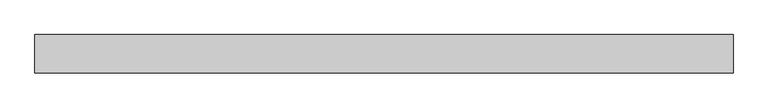
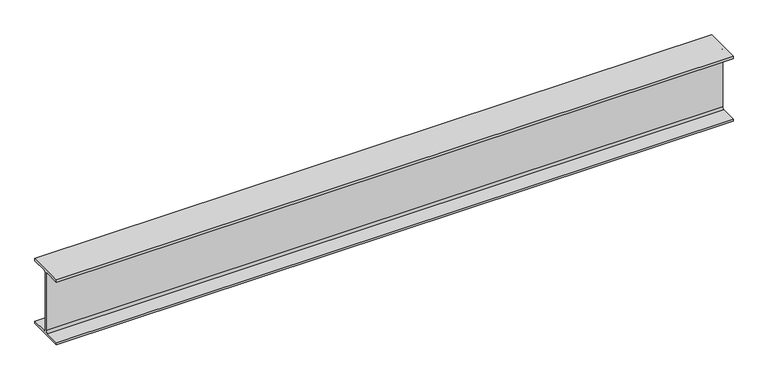
"""IFC4 building model written with IfcOpenShell, lengths in millimetres: beam geometry, Steel Beam_H-KSD3502 : H_SB_ASB_H-250x125x6x9."""

import ifcopenshell
import ifcopenshell.guid

model = None  # the IFC model being written
_history = None  # IfcOwnerHistory: only IFC2X3 demands one
_inside = {}  # id of a spatial element -> (the spatial element, [elements in it])
_under = {}  # id of a project, library or spatial element -> (it, [spatial elements below it])
_declared = {}  # id of a project -> (the project, [libraries it declares])
_typed = {}  # id of a type object -> (the type object, [elements of that type])
_made_of = {}  # id of a material, layer set ... -> (it, [elements and type objects made of it])


def new_model(schema):
    """Start an empty IFC model of exactly this schema.

    Asked for "IFC4X3", IfcOpenShell would pick the latest addendum, in which some entities
    have other attributes; the version numbers below select the first issue.
    IFC2X3 requires an IfcOwnerHistory on every rooted entity: one is made here for all.
    """
    global model, _history
    if schema == "IFC4X3":
        model = ifcopenshell.file(schema_version=(4, 3, 0, 0))
    else:
        model = ifcopenshell.file(schema=schema)
    _inside.clear()
    _under.clear()
    _declared.clear()
    _typed.clear()
    _made_of.clear()
    _history = None
    if model.schema == "IFC2X3":
        org = make("IfcOrganization", Name="unknown")
        user = make(
            "IfcPersonAndOrganization",
            ThePerson=make("IfcPerson", FamilyName="unknown"),
            TheOrganization=org,
        )
        app = make(
            "IfcApplication",
            ApplicationDeveloper=org,
            Version="unknown",
            ApplicationFullName="unknown",
            ApplicationIdentifier="unknown",
        )
        _history = make(
            "IfcOwnerHistory",
            OwningUser=user,
            OwningApplication=app,
            ChangeAction="ADDED",
            CreationDate=0,
        )
    return model


def make(cls, **values):
    """One entity of the class cls with the attributes given. An attribute that is None is left unset."""
    return model.create_entity(
        cls, **{name: value for name, value in values.items() if value is not None}
    )


def rooted(cls, **values):
    """An entity with a GlobalId (a new one), such as an element, a storey or a relation."""
    return make(cls, GlobalId=ifcopenshell.guid.new(), OwnerHistory=_history, **values)


def si_unit(unit_type, name, prefix=None):
    """IfcSIUnit, for example si_unit("LENGTHUNIT", "METRE", prefix="MILLI")."""
    return make("IfcSIUnit", UnitType=unit_type, Prefix=prefix, Name=name)


def assignment(units):
    """IfcUnitAssignment: the units of a project."""
    return None if units is None else make("IfcUnitAssignment", Units=units)


def point(xyz):
    """IfcCartesianPoint."""
    return None if xyz is None else make("IfcCartesianPoint", Coordinates=xyz)


def direction(xyz):
    """IfcDirection."""
    return None if xyz is None else make("IfcDirection", DirectionRatios=xyz)


def frame(location, z_axis=None, x_axis=None):
    """IfcAxis2Placement3D, a coordinate frame: its origin and axes. An axis left out is left unset."""
    return make(
        "IfcAxis2Placement3D",
        Location=point(location),
        Axis=direction(z_axis),
        RefDirection=direction(x_axis),
    )


def frame_2d(location, x_axis=None):
    """IfcAxis2Placement2D, a coordinate frame in the plane: its origin and x axis."""
    return make(
        "IfcAxis2Placement2D", Location=point(location), RefDirection=direction(x_axis)
    )


def origin():
    """The frame at (0, 0, 0) with its axes left unset."""
    return frame((0.0, 0.0, 0.0))


def place(relative_to, where):
    """IfcLocalPlacement: puts the frame where relative to a parent placement (None: the world)."""
    return make(
        "IfcLocalPlacement", PlacementRelTo=relative_to, RelativePlacement=where
    )


def context(
    kind, dimensions, precision=None, world=None, true_north=None, identifier=None
):
    """IfcGeometricRepresentationContext, for example the 3D "Model" context."""
    return make(
        "IfcGeometricRepresentationContext",
        ContextIdentifier=identifier,
        ContextType=kind,
        CoordinateSpaceDimension=dimensions,
        Precision=precision,
        WorldCoordinateSystem=world,
        TrueNorth=true_north,
    )


def project(units=None, contexts=None):
    """IfcProject with its units and contexts."""
    return rooted(
        "IfcProject",
        Name="project",
        RepresentationContexts=contexts,
        UnitsInContext=assignment(units),
    )


def spatial(cls, under=None, at=None, **own):
    """A site, building, storey or space (cls), placed at a placement, below another one or the project."""
    s = rooted(cls, ObjectPlacement=at, **own)
    if under is not None:
        _under.setdefault(under.id(), (under, []))[1].append(s)
    return s


def polyline(points):
    """IfcPolyline through the points."""
    return make("IfcPolyline", Points=[point(p) for p in points])


def circle_curve(where, radius):
    """IfcCircle in the frame where."""
    return make("IfcCircle", Position=where, Radius=radius)


def trimmed(basis, trim1, trim2, sense, master):
    """IfcTrimmedCurve: the piece of a basis curve between two trims."""
    return make(
        "IfcTrimmedCurve",
        BasisCurve=basis,
        Trim1=trim1,
        Trim2=trim2,
        SenseAgreement=sense,
        MasterRepresentation=master,
    )


def segment(curve, same_sense, transition):
    """IfcCompositeCurveSegment."""
    return make(
        "IfcCompositeCurveSegment",
        Transition=transition,
        SameSense=same_sense,
        ParentCurve=curve,
    )


def composite_curve(segments, self_intersect=None):
    """IfcCompositeCurve: segments joined end to end."""
    return make("IfcCompositeCurve", Segments=segments, SelfIntersect=self_intersect)


def outline(outer, holes=None, kind="AREA"):
    """IfcArbitraryClosedProfileDef: a profile drawn as a closed curve; with holes, ...WithVoids."""
    if holes is None:
        return make("IfcArbitraryClosedProfileDef", ProfileType=kind, OuterCurve=outer)
    return make(
        "IfcArbitraryProfileDefWithVoids",
        ProfileType=kind,
        OuterCurve=outer,
        InnerCurves=holes,
    )


def extrude(swept, where, along, depth):
    """IfcExtrudedAreaSolid: the profile swept, set in the frame where, extruded along a direction by depth."""
    return make(
        "IfcExtrudedAreaSolid",
        SweptArea=swept,
        Position=where,
        ExtrudedDirection=direction(along),
        Depth=depth,
    )


def shape(context_of_items, identifier, shape_type, items):
    """IfcShapeRepresentation: the items that make up one representation, for example the "Body"."""
    return make(
        "IfcShapeRepresentation",
        ContextOfItems=context_of_items,
        RepresentationIdentifier=identifier,
        RepresentationType=shape_type,
        Items=items,
    )


def source(mapping_origin, context_of_items, identifier, shape_type, items):
    """IfcRepresentationMap: a shape defined once, which mapped items show again and again."""
    return make(
        "IfcRepresentationMap",
        MappingOrigin=mapping_origin,
        MappedRepresentation=shape(context_of_items, identifier, shape_type, items),
    )


def transform(
    local_origin,
    x_axis=None,
    y_axis=None,
    z_axis=None,
    scale=None,
    scale2=None,
    scale3=None,
    uniform=True,
):
    """IfcCartesianTransformationOperator3D, or its non-uniform kind. x_axis, y_axis, z_axis: its Axis1, 2, 3."""
    if uniform:
        return make(
            "IfcCartesianTransformationOperator3D",
            Axis1=direction(x_axis),
            Axis2=direction(y_axis),
            LocalOrigin=point(local_origin),
            Scale=scale,
            Axis3=direction(z_axis),
        )
    return make(
        "IfcCartesianTransformationOperator3DnonUniform",
        Axis1=direction(x_axis),
        Axis2=direction(y_axis),
        LocalOrigin=point(local_origin),
        Scale=scale,
        Axis3=direction(z_axis),
        Scale2=scale2,
        Scale3=scale3,
    )


def mapped(mapping_source, mapping_target):
    """IfcMappedItem: shows the shape of a source again, moved by a transform."""
    return make(
        "IfcMappedItem", MappingSource=mapping_source, MappingTarget=mapping_target
    )


def made_of(thing, what):
    """Note that an element or type object is made of a material, layer set ...; save() writes the relation."""
    if what is not None:
        _made_of.setdefault(what.id(), (what, []))[1].append(thing)
    return thing


def element(
    cls,
    number,
    at=None,
    inside=None,
    cuts=None,
    type_object=None,
    material=None,
    context=None,
    identifier="Body",
    shape_type=None,
    held_by="IfcProductDefinitionShape",
    body=None,
    shapes=None,
    **own,
):
    """One element of the class cls, such as IfcWall. Its Tag is "e" and its number.

    at: its placement. inside: the storey or other place that contains it. cuts: it is an
    opening in that element (IfcRelVoidsElement). A single representation is given by context,
    identifier, shape_type and body (its items); several are given by shapes. held_by: the class
    of the entity that holds the representations. save() writes the other relations.
    """
    e = rooted(cls, Tag="e%d" % number, ObjectPlacement=at, **own)
    if body is not None:
        shapes = [shape(context, identifier, shape_type, body)]
    if shapes is not None:
        e.Representation = make(held_by, Representations=shapes)
    if inside is not None:
        _inside.setdefault(inside.id(), (inside, []))[1].append(e)
    if cuts is not None:
        rooted(
            "IfcRelVoidsElement", RelatingBuildingElement=cuts, RelatedOpeningElement=e
        )
    if type_object is not None:
        _typed.setdefault(type_object.id(), (type_object, []))[1].append(e)
    return made_of(e, material)


def aggregate(whole, parts):
    """IfcRelAggregates: a whole, such as a stair, and the parts it consists of."""
    return rooted("IfcRelAggregates", RelatingObject=whole, RelatedObjects=parts)


def save(model, path):
    """Write the relations noted so far, then the file.

    IfcRelAggregates (storeys below a building ...), IfcRelContainedInSpatialStructure (elements
    in a storey), IfcRelDefinesByType, IfcRelAssociatesMaterial and IfcRelDeclares: one each for
    every whole, place, type object, material and project.
    """
    for whole, parts in _under.values():
        aggregate(whole, parts)
    for where, things in _inside.values():
        rooted(
            "IfcRelContainedInSpatialStructure",
            RelatedElements=things,
            RelatingStructure=where,
        )
    for kind, things in _typed.values():
        rooted("IfcRelDefinesByType", RelatedObjects=things, RelatingType=kind)
    for what, things in _made_of.values():
        rooted("IfcRelAssociatesMaterial", RelatedObjects=things, RelatingMaterial=what)
    for by, libraries in _declared.values():
        rooted("IfcRelDeclares", RelatingContext=by, RelatedDefinitions=libraries)
    model.write(path)


def beam_841f7af1(model_context):
    return source(origin(), model_context, "Body", "SweptSolid", [
        extrude(outline(composite_curve([segment(polyline([(82.5, -141.5), (82.5, -151.7), (-82.5, -151.7), (-82.5, -141.5), (-11.9, -141.5)]), True, "CONTINUOUS"), segment(trimmed(circle_curve(frame_2d((-11.9, -132.6)), 8.9), [point((-11.9, -141.5))], [point((-3.0, -132.6))], True, "CARTESIAN"), True, "CONTINUOUS"), segment(polyline([(-3.0, -132.6), (-3.0, 132.6)]), True, "CONTINUOUS"), segment(trimmed(circle_curve(frame_2d((-11.9, 132.6)), 8.9), [point((-3.0, 132.6))], [point((-11.9, 141.5))], True, "CARTESIAN"), True, "CONTINUOUS"), segment(polyline([(-11.9, 141.5), (-82.5, 141.5), (-82.5, 151.7), (82.5, 151.7), (82.5, 141.5), (11.9, 141.5)]), True, "CONTINUOUS"), segment(trimmed(circle_curve(frame_2d((11.9, 132.6)), 8.9), [point((11.9, 141.5))], [point((3.0, 132.6))], True, "CARTESIAN"), True, "CONTINUOUS"), segment(polyline([(3.0, 132.6), (3.0, -132.6)]), True, "CONTINUOUS"), segment(trimmed(circle_curve(frame_2d((11.9, -132.6)), 8.9), [point((3.0, -132.6))], [point((11.9, -141.5))], True, "CARTESIAN"), True, "CONTINUOUS"), segment(polyline([(11.9, -141.5), (82.5, -141.5)]), True, "CONTINUOUS")], self_intersect=False)), frame((-1493.3, 0.0, 0.0), z_axis=(1.0, 0.0, 0.0), x_axis=(0.0, 1.0, 0.0)), (0.0, 0.0, 1.0), 2987.8360727),
    ])


if __name__ == "__main__":
    model = new_model("IFC4")
    model_context = context("Model", 3, world=origin())
    ifc_project = project(units=[si_unit("LENGTHUNIT", "METRE", prefix="MILLI")], contexts=[model_context])
    site = spatial("IfcSite", under=ifc_project)
    building = spatial("IfcBuilding", under=site)
    placement = place(None, origin())
    beam_shape = beam_841f7af1(model_context)
    element("IfcBeam", 1, ObjectType="Steel Beam_H-KSD3502 : H_SB_ASB_H-250x125x6x9", at=placement, inside=building, context=model_context, shape_type="MappedRepresentation", body=[
        mapped(beam_shape, transform((0.0, 0.0, 0.0), x_axis=(1.0, 0.0, 0.0), y_axis=(0.0, 1.0, 0.0), z_axis=(0.0, 0.0, 1.0))),
    ])
    save(model, "model.ifc")

# Revit data of these elements
# Type "Steel Beam_H-KSD3502 : H_SB_ASB_H-250x125x6x9"
#   Width = 12.5 cm
#   Web Thickness = 0.6 cm
#   Web Fillet = 1.2 cm
#   Warping Constant = 42539.8 cm⁶
#   Torsional Moment of Inertia = 7.8102 cm⁴
#   Torsional Modulus = 1.0 cm³
#   Section Area = 37.66 cm²
#   Plastic Modulus weak axis = 73.1 cm³
#   Plastic Modulus strong axis = 366.0 cm³
#   Perimeter = 0.97 m²/m
#   Nominal Weight = 29.60 kgf/m
#   Moment of Inertia weak axis = 294.00 cm⁴
#   Moment of Inertia strong axis = 4050.00 cm⁴
#   Height = 25.0 cm
#   Flange Thickness = 0.9 cm
#   Elastic Modulus weak axis = 47.0 cm³
#   Elastic Modulus strong axis = 324.0 cm³
#   Centroid Vertical = 12.5 cm
#   Centroid Horizontal = 6.25 cm
#   Length [instance default] = 1.5240 m
#   Structural Material [instance default] = Steel, 45-345
#   Assembly Code = ""
# Element 1 (IfcBeam, "Steel Beam_H-KSD3502 : H_SB_ASB_H-250x125x6x9")
#   Structural Material = none
# Materials
#   "Steel, 45-345": class "Metal", colour RGB 189 187 185, transparency 0, Description = "Steel 345 MPa", Cost = 0
